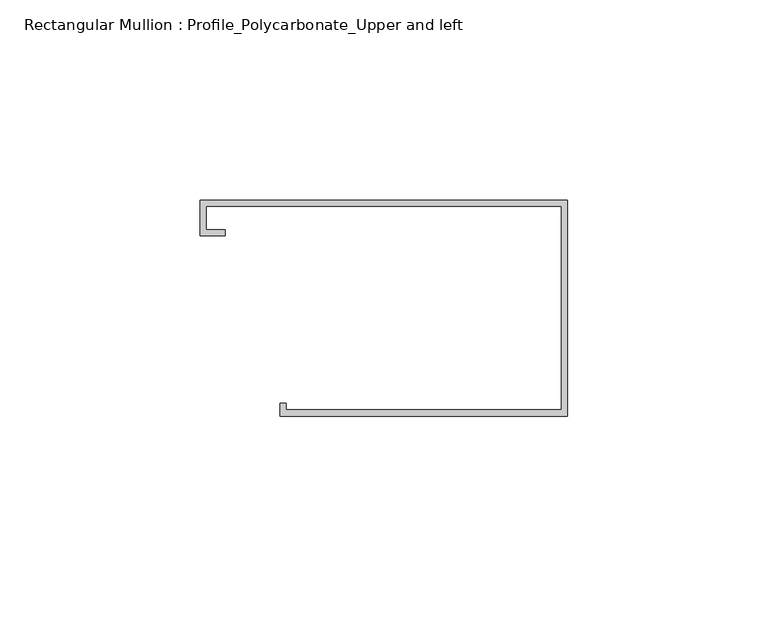
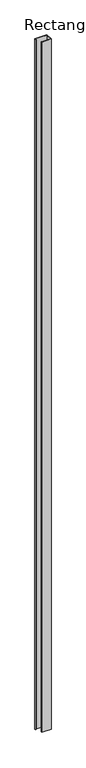
"""IFC4 building model written with IfcOpenShell, lengths in millimetres: member geometry, Rectangular Mullion : Profile_Polycarbonate_Upper and left."""

from ifc_helpers import new_model, si_unit, frame, origin, place, context, project, spatial, polyline, outline, extrude, source, transform, mapped, element, save


def rectangular_mullion_profile_polycarbonate_upper_and_left_0cf9e7c6(model_context):
    return source(origin(), model_context, "Body", "SweptSolid", [
        extrude(outline(polyline([(0.0, 28.984575), (0.0, -25.015825), (-71.9836, -25.015825), (-71.9836, -21.840825), (-70.3961, -21.840825), (-70.3961, -23.428325), (-1.5875, -23.428325), (-1.5875, 27.397075), (-90.4113, 27.397075), (-90.4113, 21.580475), (-85.6488, 21.580475), (-85.6488, 19.992975), (-91.9988, 19.992975), (-91.9988, 28.984575), (0.0, 28.984575)])), frame((0.0, 0.0, -5565.9274), z_axis=(0.0, 0.0, 1.0), x_axis=(1.0, 0.0, 0.0)), (0.0, 0.0, 1.0), 5565.9274),
    ])


if __name__ == "__main__":
    model = new_model("IFC4")
    model_context = context("Model", 3, world=origin())
    ifc_project = project(units=[si_unit("LENGTHUNIT", "METRE", prefix="MILLI")], contexts=[model_context])
    site = spatial("IfcSite", under=ifc_project)
    building = spatial("IfcBuilding", under=site)
    placement = place(None, origin())
    rectangular_mullion_profile_polycarbonate_upper_and_left_shape = rectangular_mullion_profile_polycarbonate_upper_and_left_0cf9e7c6(model_context)
    element("IfcMember", 1, ObjectType="Rectangular Mullion : Profile_Polycarbonate_Upper and left", at=placement, inside=building, context=model_context, shape_type="MappedRepresentation", body=[
        mapped(rectangular_mullion_profile_polycarbonate_upper_and_left_shape, transform((0.0, 0.0, 0.0), x_axis=(1.0, 0.0, 0.0), y_axis=(0.0, 1.0, 0.0), z_axis=(0.0, 0.0, 1.0))),
    ])
    save(model, "model.ifc")

# Revit data of these elements
# Type "Rectangular Mullion : Profile_Polycarbonate_Upper and left"
#   built-in parameter 1007322 = 0.177167 (stored number, unit not read)
#   built-in parameter 1007321 = 0.00520833 (stored number, unit not read)
#   built-in parameter 1007320 = 0 (stored number, unit not read)
